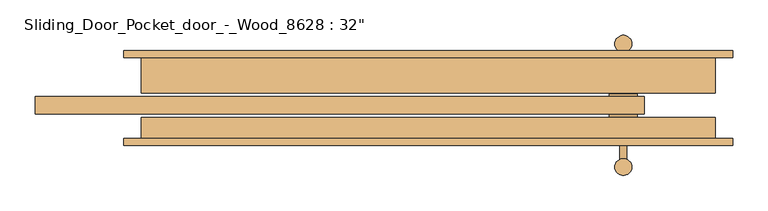
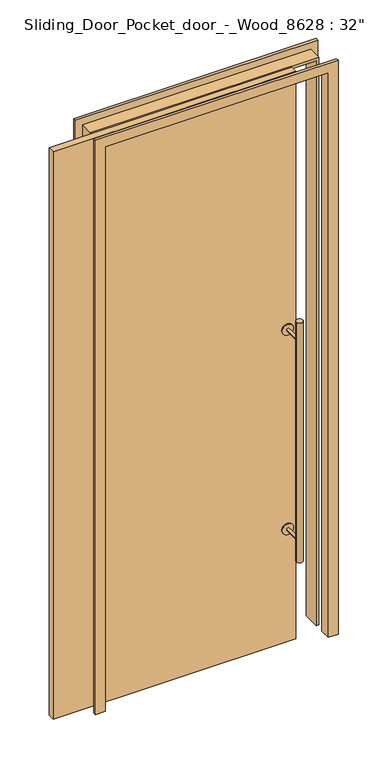
"""IFC4 building model written with IfcOpenShell, lengths in millimetres: door geometry."""

from ifc_helpers import new_model, si_unit, point, frame, frame_2d, origin, origin_with_axes, place, context, project, spatial, polyline, circle_curve, trimmed, segment, composite_curve, outline, extrude, faceted_brep, source, transform, mapped, element, save


def door_6a4a941d(model_context):
    return source(origin(), model_context, "Body", "SolidModel", [
        extrude(outline(composite_curve([segment(trimmed(circle_curve(frame_2d((256.4, 91.4218247)), 12.0), [point((244.4, 91.4218247))], [point((268.4, 91.4218247))], False, "CARTESIAN"), True, "CONTINUOUS"), segment(trimmed(circle_curve(frame_2d((256.4, 91.4218247)), 12.0), [point((268.4, 91.4218247))], [point((244.4, 91.4218247))], False, "CARTESIAN"), True, "CONTINUOUS")], self_intersect=False)), frame((0.0, 0.0, 350.0), z_axis=(0.0, 0.0, 1.0), x_axis=(1.0, 0.0, 0.0)), (0.0, 0.0, 1.0), 900.0),
        extrude(outline(composite_curve([segment(trimmed(circle_curve(frame_2d((1175.0, 256.4)), 5.0), [point((1175.0, 261.4))], [point((1175.0, 251.4))], False, "CARTESIAN"), True, "CONTINUOUS"), segment(trimmed(circle_curve(frame_2d((1175.0, 256.4)), 5.0), [point((1175.0, 251.4))], [point((1175.0, 261.4))], False, "CARTESIAN"), True, "CONTINUOUS")], self_intersect=False)), frame((0.0, 20.4218247, 0.0), z_axis=(0.0, 1.0, 0.0), x_axis=(0.0, 0.0, 1.0)), (0.0, 0.0, 1.0), 71.0),
        extrude(outline(composite_curve([segment(trimmed(circle_curve(frame_2d((425.0, 256.4)), 5.0), [point((425.0, 261.4))], [point((425.0, 251.4))], False, "CARTESIAN"), True, "CONTINUOUS"), segment(trimmed(circle_curve(frame_2d((425.0, 256.4)), 5.0), [point((425.0, 251.4))], [point((425.0, 261.4))], False, "CARTESIAN"), True, "CONTINUOUS")], self_intersect=False)), frame((0.0, 20.4218247, 0.0), z_axis=(0.0, 1.0, 0.0), x_axis=(0.0, 0.0, 1.0)), (0.0, 0.0, 1.0), 71.0),
        extrude(outline(composite_curve([segment(trimmed(circle_curve(frame_2d((1175.0, 256.4)), 20.0), [point((1175.0, 236.4))], [point((1175.0, 276.4))], False, "CARTESIAN"), True, "CONTINUOUS"), segment(trimmed(circle_curve(frame_2d((1175.0, 256.4)), 20.0), [point((1175.0, 276.4))], [point((1175.0, 236.4))], False, "CARTESIAN"), True, "CONTINUOUS")], self_intersect=False)), frame((0.0, 16.4218247, 0.0), z_axis=(0.0, 1.0, 0.0), x_axis=(0.0, 0.0, 1.0)), (0.0, 0.0, 1.0), 4.0),
        extrude(outline(composite_curve([segment(trimmed(circle_curve(frame_2d((425.0, 256.4)), 20.0), [point((425.0, 236.4))], [point((425.0, 276.4))], False, "CARTESIAN"), True, "CONTINUOUS"), segment(trimmed(circle_curve(frame_2d((425.0, 256.4)), 20.0), [point((425.0, 276.4))], [point((425.0, 236.4))], False, "CARTESIAN"), True, "CONTINUOUS")], self_intersect=False)), frame((0.0, 16.4218247, 0.0), z_axis=(0.0, 1.0, 0.0), x_axis=(0.0, 0.0, 1.0)), (0.0, 0.0, 1.0), 4.0),
        extrude(outline(composite_curve([segment(trimmed(circle_curve(frame_2d((256.4, -83.5781753)), 12.0), [point((244.4, -83.5781753))], [point((268.4, -83.5781753))], False, "CARTESIAN"), True, "CONTINUOUS"), segment(trimmed(circle_curve(frame_2d((256.4, -83.5781753)), 12.0), [point((268.4, -83.5781753))], [point((244.4, -83.5781753))], False, "CARTESIAN"), True, "CONTINUOUS")], self_intersect=False)), frame((0.0, 0.0, 350.0), z_axis=(0.0, 0.0, 1.0), x_axis=(1.0, 0.0, 0.0)), (0.0, 0.0, 1.0), 900.0),
        extrude(outline(composite_curve([segment(trimmed(circle_curve(frame_2d((1175.0, 256.4)), 5.0), [point((1175.0, 261.4))], [point((1175.0, 251.4))], False, "CARTESIAN"), True, "CONTINUOUS"), segment(trimmed(circle_curve(frame_2d((1175.0, 256.4)), 5.0), [point((1175.0, 251.4))], [point((1175.0, 261.4))], False, "CARTESIAN"), True, "CONTINUOUS")], self_intersect=False)), frame((0.0, -83.5781753, 0.0), z_axis=(0.0, 1.0, 0.0), x_axis=(0.0, 0.0, 1.0)), (0.0, 0.0, 1.0), 71.0),
        extrude(outline(composite_curve([segment(trimmed(circle_curve(frame_2d((425.0, 256.4)), 5.0), [point((425.0, 261.4))], [point((425.0, 251.4))], False, "CARTESIAN"), True, "CONTINUOUS"), segment(trimmed(circle_curve(frame_2d((425.0, 256.4)), 5.0), [point((425.0, 251.4))], [point((425.0, 261.4))], False, "CARTESIAN"), True, "CONTINUOUS")], self_intersect=False)), frame((0.0, -83.5781753, 0.0), z_axis=(0.0, 1.0, 0.0), x_axis=(0.0, 0.0, 1.0)), (0.0, 0.0, 1.0), 71.0),
        extrude(outline(composite_curve([segment(trimmed(circle_curve(frame_2d((1175.0, 256.4)), 20.0), [point((1175.0, 236.4))], [point((1175.0, 276.4))], False, "CARTESIAN"), True, "CONTINUOUS"), segment(trimmed(circle_curve(frame_2d((1175.0, 256.4)), 20.0), [point((1175.0, 276.4))], [point((1175.0, 236.4))], False, "CARTESIAN"), True, "CONTINUOUS")], self_intersect=False)), frame((0.0, -12.5781753, 0.0), z_axis=(0.0, 1.0, 0.0), x_axis=(0.0, 0.0, 1.0)), (0.0, 0.0, 1.0), 4.0),
        extrude(outline(composite_curve([segment(trimmed(circle_curve(frame_2d((425.0, 256.4)), 20.0), [point((425.0, 236.4))], [point((425.0, 276.4))], False, "CARTESIAN"), True, "CONTINUOUS"), segment(trimmed(circle_curve(frame_2d((425.0, 256.4)), 20.0), [point((425.0, 276.4))], [point((425.0, 236.4))], False, "CARTESIAN"), True, "CONTINUOUS")], self_intersect=False)), frame((0.0, -12.5781753, 0.0), z_axis=(0.0, 1.0, 0.0), x_axis=(0.0, 0.0, 1.0)), (0.0, 0.0, 1.0), 4.0),
        extrude(outline(polyline([(286.4, 16.4218247), (286.4, -8.5781753), (-576.4, -8.5781753), (-576.4, 16.4218247), (286.4, 16.4218247)])), origin_with_axes(), (0.0, 0.0, 1.0), 2133.6),
        faceted_brep([(386.4, 21.4218247, 0.0), (376.4, 21.4218247, 0.0), (376.4, 81.4218247, 0.0), (411.4, 81.4218247, 0.0), (411.4, 71.4218247, 0.0), (386.4, 71.4218247, 0.0), (386.4, 21.4218247, 2133.6), (-426.4, 21.4218247, 2133.6), (-426.4, 21.4218247, 0.0), (-416.4, 21.4218247, 0.0), (-416.4, 21.4218247, 2123.6), (376.4, 21.4218247, 2123.6), (376.4, 81.4218247, 2123.6), (-416.4, 81.4218247, 2123.6), (-416.4, 81.4218247, 0.0), (-451.4, 81.4218247, 0.0), (-451.4, 81.4218247, 2158.6), (411.4, 81.4218247, 2158.6), (411.4, 71.4218247, 2158.6), (-451.4, 71.4218247, 2158.6), (-451.4, 71.4218247, 0.0), (-426.4, 71.4218247, 0.0), (-426.4, 71.4218247, 2133.6), (386.4, 71.4218247, 2133.6)], [[[0, 1, 2, 3, 4, 5]], [[1, 0, 6, 7, 8, 9, 10, 11]], [[2, 1, 11, 12]], [[3, 2, 12, 13, 14, 15, 16, 17]], [[4, 3, 17, 18]], [[5, 4, 18, 19, 20, 21, 22, 23]], [[0, 5, 23, 6]], [[7, 22, 21, 8]], [[8, 21, 20, 15, 14, 9]], [[13, 10, 9, 14]], [[19, 16, 15, 20]], [[6, 23, 22, 7]], [[12, 11, 10, 13]], [[18, 17, 16, 19]]]),
        faceted_brep([(386.4, -13.5781753, 0.0), (386.4, -42.8781753, 0.0), (411.4, -42.8781753, 0.0), (411.4, -52.8781753, 0.0), (376.4, -52.8781753, 0.0), (376.4, -13.5781753, 0.0), (386.4, -13.5781753, 2133.6), (386.4, -42.8781753, 2133.6), (-426.4, -42.8781753, 2133.6), (-426.4, -42.8781753, 0.0), (-451.4, -42.8781753, 0.0), (-451.4, -42.8781753, 2158.6), (411.4, -42.8781753, 2158.6), (411.4, -52.8781753, 2158.6), (-451.4, -52.8781753, 2158.6), (-451.4, -52.8781753, 0.0), (-416.4, -52.8781753, 0.0), (-416.4, -52.8781753, 2123.6), (376.4, -52.8781753, 2123.6), (376.4, -13.5781753, 2123.6), (-416.4, -13.5781753, 2123.6), (-416.4, -13.5781753, 0.0), (-426.4, -13.5781753, 0.0), (-426.4, -13.5781753, 2133.6)], [[[0, 1, 2, 3, 4, 5]], [[1, 0, 6, 7]], [[2, 1, 7, 8, 9, 10, 11, 12]], [[3, 2, 12, 13]], [[4, 3, 13, 14, 15, 16, 17, 18]], [[5, 4, 18, 19]], [[0, 5, 19, 20, 21, 22, 23, 6]], [[22, 21, 16, 15, 10, 9]], [[20, 17, 16, 21]], [[8, 23, 22, 9]], [[14, 11, 10, 15]], [[7, 6, 23, 8]], [[19, 18, 17, 20]], [[13, 12, 11, 14]]]),
    ])


if __name__ == "__main__":
    model = new_model("IFC4")
    model_context = context("Model", 3, world=origin())
    ifc_project = project(units=[si_unit("LENGTHUNIT", "METRE", prefix="MILLI")], contexts=[model_context])
    site = spatial("IfcSite", under=ifc_project)
    building = spatial("IfcBuilding", under=site)
    placement = place(None, origin())
    door_shape = door_6a4a941d(model_context)
    element("IfcDoor", 1, ObjectType="Sliding_Door_Pocket_door_-_Wood_8628 : 32\"", at=placement, inside=building, context=model_context, shape_type="MappedRepresentation", body=[
        mapped(door_shape, transform((0.0, 0.0, 0.0), x_axis=(1.0, 0.0, 0.0), y_axis=(0.0, 1.0, 0.0), z_axis=(0.0, 0.0, 1.0))),
    ])
    save(model, "model.ifc")

# Revit data of these elements
# Type "Sliding_Door_Pocket_door_-_Wood_8628 : 32\""
#   Type Mark = "45"
#   Frame Projection Ext. = 0' - 0.98425"
#   Frame Projection Int. = 0' - 0.98425"
#   Frame Width = 0' - 2.95276"
#   Height = 7' - 0"
#   Width = 2' - 8"
#   Espessura Porta = 0' - 1.37795"
#   Dist_Porta = 0' - 1.9685"
#   Comp_Painel = 2' - 9.9685"
#   Abertura [instance default] = 0' - 3.93701"
#   A [instance default] = 0' - 3.93701"
#   Material Painel [instance default] = Porta_Material
#   Material Aro = Porta_Material
#   Function = (empty or 0)
#   Wall Closure = (empty or 0)
# Element 1 (IfcDoor, "Sliding_Door_Pocket_door_-_Wood_8628 : 32\"")
#   Materials on its faces: "Ironmongery - SS", "Porta_Material"
# Materials
#   "Porta_Material": class "Wood", colour RGB 129 89 45, transparency 0
#   "Ironmongery - SS": class "Miscellaneous", colour RGB 247 247 247, transparency 0
